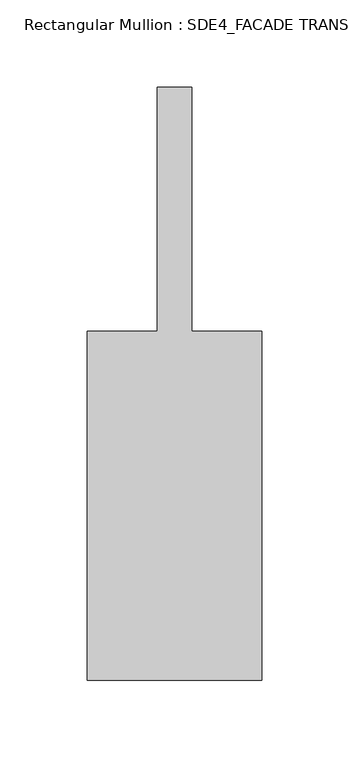
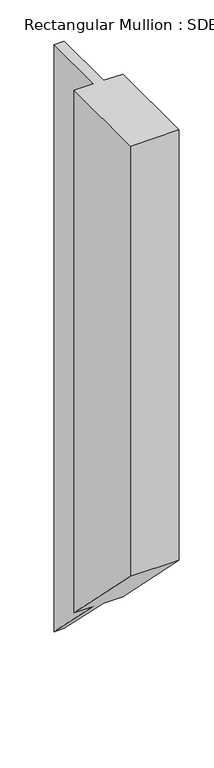
"""IFC4 building model written with IfcOpenShell, lengths in millimetres: member geometry, Rectangular Mullion : SDE4_FACADE TRANSOM TYPE 1."""

from ifc_helpers import new_model, si_unit, origin, place, context, project, spatial, faceted_brep, source, transform, mapped, element, save


def rectangular_mullion_sde4_facade_transom_type_1_fd896079(model_context):
    return source(origin(), model_context, "Body", "Brep", [
        faceted_brep([(50.0, -132.5, 0.0), (50.0, 67.5, 0.0), (10.0, 67.5, 0.0), (10.0, 207.5, 0.0), (-10.0, 207.5, 0.0), (-10.0, 67.5, 0.0), (-50.0, 67.5, 0.0), (-50.0, -132.5, 0.0), (50.0, -132.5, -933.9624711), (50.0, 67.5, -1133.9624711), (10.0, 67.5, -1133.9624711), (10.0, 207.5, -1273.9624711), (-10.0, 207.5, -1273.9624711), (-10.0, 67.5, -1133.9624711), (-50.0, 67.5, -1133.9624711), (-50.0, -132.5, -933.9624711)], [[[0, 1, 2, 3, 4, 5, 6, 7]], [[1, 0, 8, 9]], [[2, 1, 9, 10]], [[3, 2, 10, 11]], [[4, 3, 11, 12]], [[5, 4, 12, 13]], [[6, 5, 13, 14]], [[7, 6, 14, 15]], [[0, 7, 15, 8]], [[8, 15, 14, 13, 12, 11, 10, 9]]]),
    ])


if __name__ == "__main__":
    model = new_model("IFC4")
    model_context = context("Model", 3, world=origin())
    ifc_project = project(units=[si_unit("LENGTHUNIT", "METRE", prefix="MILLI")], contexts=[model_context])
    site = spatial("IfcSite", under=ifc_project)
    building = spatial("IfcBuilding", under=site)
    placement = place(None, origin())
    rectangular_mullion_sde4_facade_transom_type_1_shape = rectangular_mullion_sde4_facade_transom_type_1_fd896079(model_context)
    element("IfcMember", 1, ObjectType="Rectangular Mullion : SDE4_FACADE TRANSOM TYPE 1", at=placement, inside=building, context=model_context, shape_type="MappedRepresentation", body=[
        mapped(rectangular_mullion_sde4_facade_transom_type_1_shape, transform((0.0, 0.0, 0.0), x_axis=(1.0, 0.0, 0.0), y_axis=(0.0, 1.0, 0.0), z_axis=(0.0, 0.0, 1.0))),
    ])
    save(model, "model.ifc")

# Revit data of these elements
# Type "Rectangular Mullion : SDE4_FACADE TRANSOM TYPE 1"
#   built-in parameter 1007322 = 1.11549 (stored number, unit not read)
#   built-in parameter 1007321 = 0.164042 (stored number, unit not read)
#   built-in parameter 1007320 = 0.164042 (stored number, unit not read)
